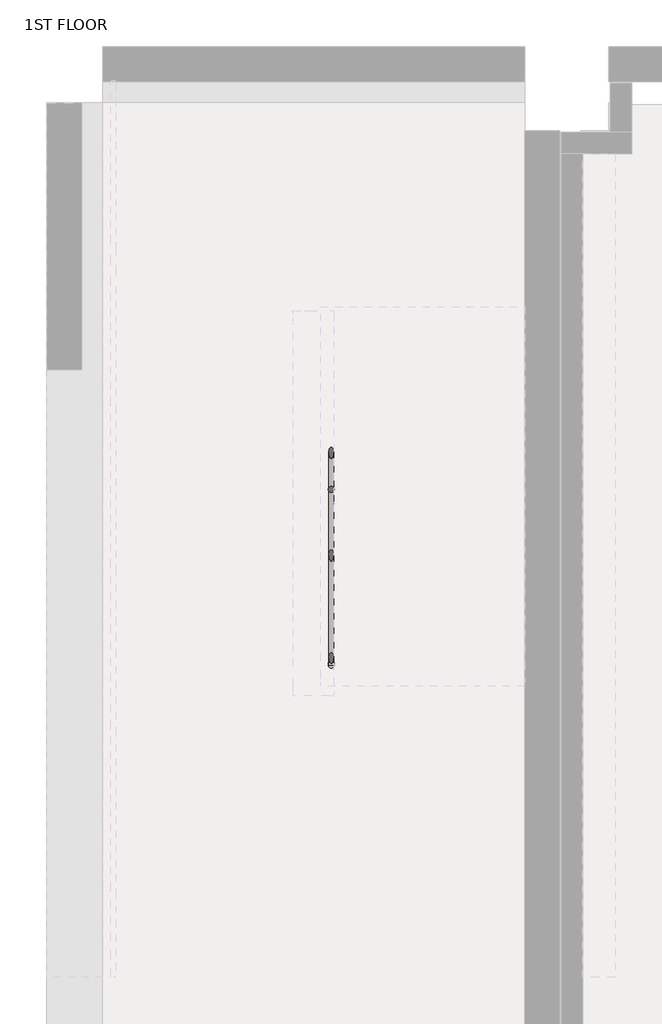
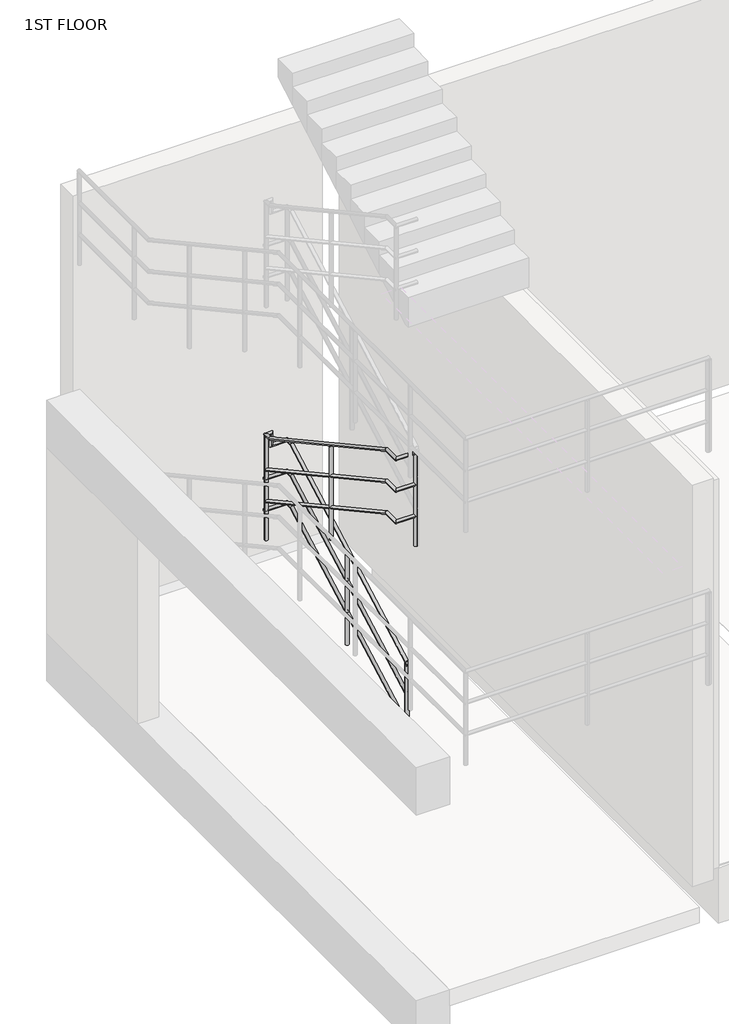
# One storey, part 12 of 15: 1 railing.
"""IFC4 building model written with IfcOpenShell, lengths in millimetres."""

from ifc_helpers import new_model, si_unit, point, frame, frame_2d, origin, place, context, project, spatial, circle_curve, ellipse_curve, trimmed, segment, composite_curve, outline, extrude, element, save
from ifc_brep_helpers import plane_surface, cylinder_surface, advanced_brep

model = new_model("IFC4")

# Units and contexts
model_context = context("Model", 3, world=origin())
ifc_project = project(units=[si_unit("LENGTHUNIT", "METRE", prefix="MILLI")], contexts=[model_context])

# Site, building, storey
site = spatial("IfcSite", under=ifc_project)
building = spatial("IfcBuilding", under=site)
storey = spatial("IfcBuildingStorey", under=building, Name="1ST FLOOR", Elevation=4800.0)

# Railing
placement = place(None, origin())
element("IfcRailing", 1, ObjectType="H_RL_AR_S10_Steel Handrail_H1200_STAIR", at=placement, inside=storey, context=model_context, shape_type="SolidModel", body=[
    advanced_brep(
    [(-1656.0, -4100.0, 5972.7772257), (-1694.0, -4100.0, 5972.7772257), (-1656.0, -1695.134128, 7291.0), (-1694.0, -1695.134128, 7291.0), (-1656.0, -1581.0, 7291.0), (-1694.0, -1619.0, 7291.0), (-1868.0, -1581.0, 7291.0), (-1868.0, -1619.0, 7291.0), (-1868.0, -1581.0, 7442.2888889), (-1868.0, -1619.0, 7442.2888889), (-1944.0, -1581.0, 7442.2888889), (-1906.0, -1619.0, 7442.2888889), (-1944.0, -1680.865872, 7442.2888889), (-1906.0, -1680.865872, 7442.2888889), (-1944.0, -4104.865872, 8771.0), (-1906.0, -4104.865872, 8771.0), (-1944.0, -4319.0, 8771.0), (-1906.0, -4281.0, 8771.0), (-1675.0, -4319.0, 8771.0), (-1675.0, -4281.0, 8771.0)],
    [
        (0, 1, ellipse_curve(frame((-1675.0, -4100.0, 5972.7772257), z_axis=(0.0, -1.0, 0.0), x_axis=(0.0, 0.0, -0.9999999999999999)), 21.6672187, 19.0)),
        (1, 0, ellipse_curve(frame((-1675.0, -4100.0, 5972.7772257), z_axis=(0.0, -1.0, 0.0), x_axis=(0.0, 0.0, -0.9999999999999999)), 21.6672187, 19.0)),
        (0, 2),
        (2, 3, ellipse_curve(frame((-1675.0, -1695.134128, 7291.0), z_axis=(0.0, -0.9687364795192939, -0.24809198545814526), x_axis=(0.0, 0.2480919854581443, -0.9687364795192942)), 19.613177, 19.0)),
        (3, 1),
        (3, 2, ellipse_curve(frame((-1675.0, -1695.134128, 7291.0), z_axis=(0.0, -0.9687364795192939, -0.24809198545814526), x_axis=(0.0, 0.2480919854581443, -0.9687364795192942)), 19.613177, 19.0)),
        (2, 4),
        (4, 5, ellipse_curve(frame((-1675.0, -1600.0, 7291.0), z_axis=(0.7071067811865467, -0.7071067811865485, 0.0), x_axis=(-0.7071067811865485, -0.7071067811865465, 0.0)), 26.8700577, 19.0)),
        (5, 3),
        (5, 4, ellipse_curve(frame((-1675.0, -1600.0, 7291.0), z_axis=(0.7071067811865467, -0.7071067811865485, 0.0), x_axis=(-0.7071067811865485, -0.7071067811865465, 0.0)), 26.8700577, 19.0)),
        (4, 6),
        (6, 7, ellipse_curve(frame((-1868.0, -1600.0, 7291.0), z_axis=(0.7071067811865475, 0.0, -0.7071067811865475), x_axis=(0.7071067811865476, 0.0, 0.7071067811865474)), 26.8700577, 19.0)),
        (7, 5),
        (7, 6, ellipse_curve(frame((-1868.0, -1600.0, 7291.0), z_axis=(0.7071067811865475, 0.0, -0.7071067811865475), x_axis=(0.7071067811865476, 0.0, 0.7071067811865474)), 26.8700577, 19.0)),
        (6, 8),
        (8, 9, ellipse_curve(frame((-1868.0, -1600.0, 7442.2888889), z_axis=(0.7071067811865475, 0.0, -0.7071067811865475), x_axis=(-0.7071067811865474, 0.0, -0.7071067811865476)), 26.8700577, 19.0)),
        (9, 7),
        (9, 8, ellipse_curve(frame((-1868.0, -1600.0, 7442.2888889), z_axis=(0.7071067811865475, 0.0, -0.7071067811865475), x_axis=(-0.7071067811865474, 0.0, -0.7071067811865476)), 26.8700577, 19.0)),
        (8, 10),
        (10, 11, ellipse_curve(frame((-1925.0, -1600.0, 7442.2888889), z_axis=(0.70710678118664, 0.707106781186455, 0.0), x_axis=(0.707106781186455, -0.70710678118664, 0.0)), 26.8700577, 19.0)),
        (11, 9),
        (11, 10, ellipse_curve(frame((-1925.0, -1600.0, 7442.2888889), z_axis=(0.70710678118664, 0.707106781186455, 0.0), x_axis=(0.707106781186455, -0.70710678118664, 0.0)), 26.8700577, 19.0)),
        (10, 12),
        (12, 13, ellipse_curve(frame((-1925.0, -1680.865872, 7442.2888889), z_axis=(0.0, 0.9687364795192939, -0.24809198545814531), x_axis=(0.0, 0.24809198545814604, 0.9687364795192938)), 19.613177, 19.0)),
        (13, 11),
        (13, 12, ellipse_curve(frame((-1925.0, -1680.865872, 7442.2888889), z_axis=(0.0, 0.9687364795192939, -0.24809198545814531), x_axis=(0.0, 0.24809198545814604, 0.9687364795192938)), 19.613177, 19.0)),
        (12, 14),
        (14, 15, ellipse_curve(frame((-1925.0, -4104.865872, 8771.0), z_axis=(0.0, 0.9687364795192939, -0.2480919854581453), x_axis=(0.0, -0.24809198545814418, -0.9687364795192942)), 19.613177, 19.0)),
        (15, 13),
        (15, 14, ellipse_curve(frame((-1925.0, -4104.865872, 8771.0), z_axis=(0.0, 0.9687364795192939, -0.2480919854581453), x_axis=(0.0, -0.24809198545814418, -0.9687364795192942)), 19.613177, 19.0)),
        (14, 16),
        (16, 17, ellipse_curve(frame((-1925.0, -4300.0, 8771.0), z_axis=(-0.7071067811864243, 0.7071067811866708, 0.0), x_axis=(0.7071067811866707, 0.7071067811864242, 0.0)), 26.8700577, 19.0)),
        (17, 15),
        (17, 16, ellipse_curve(frame((-1925.0, -4300.0, 8771.0), z_axis=(-0.7071067811864243, 0.7071067811866708, 0.0), x_axis=(0.7071067811866707, 0.7071067811864242, 0.0)), 26.8700577, 19.0)),
        (18, 19, circle_curve(frame((-1675.0, -4300.0, 8771.0), z_axis=(1.0, 0.0, 0.0), x_axis=(0.0, 1.0, 0.0)), 19.0)),
        (19, 18, circle_curve(frame((-1675.0, -4300.0, 8771.0), z_axis=(1.0, 0.0, 0.0), x_axis=(0.0, 1.0, 0.0)), 19.0)),
        (16, 18),
        (19, 17),
    ],
    [
        plane_surface(frame((-1675.0, -4100.0, 5994.4444444), z_axis=(0.0, -1.0, 0.0), x_axis=(0.0, 0.0, 1.0))),
        cylinder_surface(frame((-1675.0, -4090.8672412, 5977.7833305), z_axis=(0.0, -0.8769007335028709, -0.4806715131793511), x_axis=(-1.0, 0.0, 0.0)), 19.0),
        cylinder_surface(frame((-1675.0, -1700.0, 7291.0), z_axis=(0.0, -1.0, 0.0), x_axis=(-1.0, 0.0, 0.0)), 19.0),
        cylinder_surface(frame((-1675.0, -1600.0, 7291.0), z_axis=(1.0, 0.0, 0.0), x_axis=(0.0, -1.0, 0.0)), 19.0),
        cylinder_surface(frame((-1868.0, -1600.0, 7310.0), z_axis=(0.0, 0.0, -1.0), x_axis=(0.0, -1.0, 0.0)), 19.0),
        cylinder_surface(frame((-1849.0, -1600.0, 7442.2888889), z_axis=(1.0, 0.0, 0.0), x_axis=(0.0, -1.0, 0.0)), 19.0),
        cylinder_surface(frame((-1925.0, -1600.0, 7442.2888889), z_axis=(0.0, 1.0, 0.0), x_axis=(1.0, 0.0, 0.0)), 19.0),
        cylinder_surface(frame((-1925.0, -1685.1327588, 7444.627775), z_axis=(0.0, 0.8769007335028708, -0.4806715131793512), x_axis=(1.0, 0.0, 0.0)), 19.0),
        cylinder_surface(frame((-1925.0, -4100.0, 8771.0), z_axis=(0.0, 1.0, 0.0), x_axis=(1.0, 0.0, 0.0)), 19.0),
        plane_surface(frame((-1675.0, -4300.0, 8790.0), z_axis=(1.0, 0.0, 0.0), x_axis=(0.0, 1.0, 0.0))),
        cylinder_surface(frame((-1925.0, -4300.0, 8771.0), z_axis=(-1.0, 0.0, 0.0), x_axis=(0.0, 1.0, 0.0)), 19.0),
    ],
    [
        (0, [[1, 2]]),
        (1, [[-1, 3, 4, 5]]),
        (1, [[-2, -5, 6, -3]]),
        (2, [[-4, 7, 8, 9]]),
        (2, [[-6, -9, 10, -7]]),
        (3, [[-8, 11, 12, 13]]),
        (3, [[-10, -13, 14, -11]]),
        (4, [[-12, 15, 16, 17]]),
        (4, [[-14, -17, 18, -15]]),
        (5, [[-16, 19, 20, 21]]),
        (5, [[-18, -21, 22, -19]]),
        (6, [[-20, 23, 24, 25]]),
        (6, [[-22, -25, 26, -23]]),
        (7, [[-24, 27, 28, 29]]),
        (7, [[-26, -29, 30, -27]]),
        (8, [[-28, 31, 32, 33]]),
        (8, [[-30, -33, 34, -31]]),
        (9, [[35, 36]]),
        (10, [[-32, 37, -36, 38]]),
        (10, [[-34, -38, -35, -37]]),
    ],
),
    advanced_brep(
    [(-1675.0, -4319.0, 7971.0), (-1675.0, -4281.0, 7971.0), (-1944.0, -4319.0, 7971.0), (-1906.0, -4281.0, 7971.0)],
    [
        (0, 1, circle_curve(frame((-1675.0, -4300.0, 7971.0), z_axis=(1.0, 0.0, 0.0), x_axis=(0.0, 1.0, 0.0)), 19.0)),
        (1, 0, circle_curve(frame((-1675.0, -4300.0, 7971.0), z_axis=(1.0, 0.0, 0.0), x_axis=(0.0, 1.0, 0.0)), 19.0)),
        (2, 3, ellipse_curve(frame((-1925.0, -4300.0, 7971.0), z_axis=(-0.7071067811865471, 0.7071067811865479, 0.0), x_axis=(0.7071067811865479, 0.7071067811865471, 0.0)), 26.8700577, 19.0)),
        (3, 2, ellipse_curve(frame((-1925.0, -4300.0, 7971.0), z_axis=(-0.7071067811865471, 0.7071067811865479, 0.0), x_axis=(0.7071067811865479, 0.7071067811865471, 0.0)), 26.8700577, 19.0)),
        (0, 2),
        (3, 1),
    ],
    [
        plane_surface(frame((-1675.0, -4300.0, 7990.0), z_axis=(1.0, 0.0, 0.0), x_axis=(0.0, -1.0, 0.0))),
        plane_surface(frame((-1925.0, -4300.0, 7990.0), z_axis=(-0.7071067811865471, 0.7071067811865479, 0.0), x_axis=(0.7071067811865479, 0.7071067811865471, 0.0))),
        cylinder_surface(frame((-1675.0, -4300.0, 7971.0), z_axis=(1.0, 0.0, 0.0), x_axis=(0.0, 1.0, 0.0)), 19.0),
    ],
    [
        (0, [[1, 2]]),
        (1, [[3, 4]]),
        (2, [[-1, 5, -4, 6]]),
        (2, [[-2, -6, -3, -5]]),
    ],
),
    advanced_brep(
    [(-1944.0, -4319.0, 7971.0), (-1906.0, -4281.0, 7971.0), (-1944.0, -4104.865872, 7971.0), (-1906.0, -4104.865872, 7971.0), (-1944.0, -1592.4716448, 6593.8357569), (-1906.0, -1625.7938727, 6612.1012744)],
    [
        (0, 1, ellipse_curve(frame((-1925.0, -4300.0, 7971.0), z_axis=(0.7071067811865471, -0.7071067811865479, 0.0), x_axis=(-0.7071067811865478, -0.7071067811865472, 0.0)), 26.8700577, 19.0)),
        (1, 0, ellipse_curve(frame((-1925.0, -4300.0, 7971.0), z_axis=(0.7071067811865471, -0.7071067811865479, 0.0), x_axis=(-0.7071067811865478, -0.7071067811865472, 0.0)), 26.8700577, 19.0)),
        (0, 2),
        (2, 3, ellipse_curve(frame((-1925.0, -4104.865872, 7971.0), z_axis=(0.0, -0.9687364795192939, 0.24809198545814531), x_axis=(0.0, -0.24809198545814604, -0.9687364795192938)), 19.613177, 19.0)),
        (3, 1),
        (3, 2, ellipse_curve(frame((-1925.0, -4104.865872, 7971.0), z_axis=(0.0, -0.9687364795192939, 0.24809198545814531), x_axis=(0.0, -0.24809198545814604, -0.9687364795192938)), 19.613177, 19.0)),
        (4, 5, ellipse_curve(frame((-1925.0, -1609.1327588, 6602.9685157), z_axis=(0.7071067811865346, 0.6200624550873559, -0.33988608649231156), x_axis=(0.7071067811865606, -0.6200624550873189, 0.33988608649232477)), 26.8700577, 19.0)),
        (5, 4, ellipse_curve(frame((-1925.0, -1609.1327588, 6602.9685157), z_axis=(0.7071067811865346, 0.6200624550873559, -0.33988608649231156), x_axis=(0.7071067811865606, -0.6200624550873189, 0.33988608649232477)), 26.8700577, 19.0)),
        (2, 4),
        (5, 3),
    ],
    [
        plane_surface(frame((-1925.0, -4300.0, 7990.0), z_axis=(0.7071067811865471, -0.7071067811865479, 0.0), x_axis=(0.7071067811865479, 0.7071067811865471, 0.0))),
        cylinder_surface(frame((-1925.0, -4300.0, 7971.0), z_axis=(0.0, -1.0, 0.0), x_axis=(1.0, 0.0, 0.0)), 19.0),
        plane_surface(frame((-1925.0, -1600.0, 6619.6296296), z_axis=(0.7071067811865346, 0.6200624550873559, -0.33988608649231156), x_axis=(0.7071067811865605, -0.6200624550873332, 0.33988608649229907))),
        cylinder_surface(frame((-1925.0, -4109.1327588, 7973.3388861), z_axis=(0.0, -0.8769007335028708, 0.4806715131793512), x_axis=(1.0, 0.0, 0.0)), 19.0),
    ],
    [
        (0, [[1, 2]]),
        (1, [[-1, 3, 4, 5]]),
        (1, [[-2, -5, 6, -3]]),
        (2, [[7, 8]]),
        (3, [[-4, 9, -8, 10]]),
        (3, [[-6, -10, -7, -9]]),
    ],
),
    advanced_brep(
    [(-1950.7938727, -1581.0, 6491.0), (-1917.4716448, -1619.0, 6491.0), (-1656.0, -1581.0, 6491.0), (-1694.0, -1619.0, 6491.0)],
    [
        (0, 1, ellipse_curve(frame((-1934.1327587, -1600.0, 6491.0), z_axis=(-0.7071067811865346, -0.6200624550873559, 0.33988608649231156), x_axis=(-0.7071067811865603, 0.6200624550873332, -0.33988608649229907)), 26.8700577, 19.0)),
        (1, 0, ellipse_curve(frame((-1934.1327587, -1600.0, 6491.0), z_axis=(-0.7071067811865346, -0.6200624550873559, 0.33988608649231156), x_axis=(-0.7071067811865603, 0.6200624550873332, -0.33988608649229907)), 26.8700577, 19.0)),
        (2, 3, ellipse_curve(frame((-1675.0, -1600.0, 6491.0), z_axis=(0.7071067811865619, -0.7071067811865331, 0.0), x_axis=(-0.7071067811865331, -0.7071067811865619, 0.0)), 26.8700577, 19.0)),
        (3, 2, ellipse_curve(frame((-1675.0, -1600.0, 6491.0), z_axis=(0.7071067811865619, -0.7071067811865331, 0.0), x_axis=(-0.7071067811865331, -0.7071067811865619, 0.0)), 26.8700577, 19.0)),
        (0, 2),
        (3, 1),
    ],
    [
        plane_surface(frame((-1925.0, -1600.0, 6510.0), z_axis=(-0.7071067811865346, -0.6200624550873559, 0.33988608649231156), x_axis=(0.7071067811865605, -0.6200624550873332, 0.33988608649229907))),
        plane_surface(frame((-1675.0, -1600.0, 6510.0), z_axis=(0.7071067811865619, -0.7071067811865331, 0.0), x_axis=(0.7071067811865331, 0.7071067811865619, 0.0))),
        cylinder_surface(frame((-1925.0, -1600.0, 6491.0), z_axis=(-1.0, 0.0, 0.0), x_axis=(0.0, -1.0, 0.0)), 19.0),
    ],
    [
        (0, [[1, 2]]),
        (1, [[3, 4]]),
        (2, [[-1, 5, -4, 6]]),
        (2, [[-2, -6, -3, -5]]),
    ],
),
    advanced_brep(
    [(-1656.0, -1581.0, 6491.0), (-1694.0, -1619.0, 6491.0), (-1656.0, -1695.134128, 6491.0), (-1694.0, -1695.134128, 6491.0), (-1656.0, -4100.0, 5172.7772257), (-1694.0, -4100.0, 5172.7772257)],
    [
        (0, 1, ellipse_curve(frame((-1675.0, -1600.0, 6491.0), z_axis=(-0.7071067811865619, 0.7071067811865331, 0.0), x_axis=(0.707106781186533, 0.7071067811865619, 0.0)), 26.8700577, 19.0)),
        (1, 0, ellipse_curve(frame((-1675.0, -1600.0, 6491.0), z_axis=(-0.7071067811865619, 0.7071067811865331, 0.0), x_axis=(0.707106781186533, 0.7071067811865619, 0.0)), 26.8700577, 19.0)),
        (0, 2),
        (2, 3, ellipse_curve(frame((-1675.0, -1695.134128, 6491.0), z_axis=(0.0, 0.9687364795192939, 0.24809198545814526), x_axis=(0.0, 0.2480919854581461, -0.9687364795192938)), 19.613177, 19.0)),
        (3, 1),
        (3, 2, ellipse_curve(frame((-1675.0, -1695.134128, 6491.0), z_axis=(0.0, 0.9687364795192939, 0.24809198545814526), x_axis=(0.0, 0.2480919854581461, -0.9687364795192938)), 19.613177, 19.0)),
        (4, 5, ellipse_curve(frame((-1675.0, -4100.0, 5172.7772257), z_axis=(0.0, -1.0, 0.0), x_axis=(0.0, 0.0, 0.9999999999999999)), 21.6672187, 19.0)),
        (5, 4, ellipse_curve(frame((-1675.0, -4100.0, 5172.7772257), z_axis=(0.0, -1.0, 0.0), x_axis=(0.0, 0.0, 0.9999999999999999)), 21.6672187, 19.0)),
        (2, 4),
        (5, 3),
    ],
    [
        plane_surface(frame((-1675.0, -1600.0, 6510.0), z_axis=(-0.7071067811865619, 0.7071067811865331, 0.0), x_axis=(0.7071067811865331, 0.7071067811865619, 0.0))),
        cylinder_surface(frame((-1675.0, -1600.0, 6491.0), z_axis=(0.0, 1.0, 0.0), x_axis=(-1.0, 0.0, 0.0)), 19.0),
        plane_surface(frame((-1675.0, -4100.0, 5194.4444444), z_axis=(0.0, -1.0, 0.0), x_axis=(0.0, 0.0, -1.0))),
        cylinder_surface(frame((-1675.0, -1690.8672412, 6493.3388861), z_axis=(0.0, 0.8769007335028709, 0.4806715131793511), x_axis=(-1.0, 0.0, 0.0)), 19.0),
    ],
    [
        (0, [[1, 2]]),
        (1, [[-1, 3, 4, 5]]),
        (1, [[-2, -5, 6, -3]]),
        (2, [[7, 8]]),
        (3, [[-4, 9, -8, 10]]),
        (3, [[-6, -10, -7, -9]]),
    ],
),
    advanced_brep(
    [(-1675.0, -4319.0, 8371.0), (-1675.0, -4281.0, 8371.0), (-1944.0, -4319.0, 8371.0), (-1906.0, -4281.0, 8371.0)],
    [
        (0, 1, circle_curve(frame((-1675.0, -4300.0, 8371.0), z_axis=(1.0, 0.0, 0.0), x_axis=(0.0, 1.0, 0.0)), 19.0)),
        (1, 0, circle_curve(frame((-1675.0, -4300.0, 8371.0), z_axis=(1.0, 0.0, 0.0), x_axis=(0.0, 1.0, 0.0)), 19.0)),
        (2, 3, ellipse_curve(frame((-1925.0, -4300.0, 8371.0), z_axis=(-0.7071067811865471, 0.7071067811865479, 0.0), x_axis=(0.7071067811865479, 0.7071067811865471, 0.0)), 26.8700577, 19.0)),
        (3, 2, ellipse_curve(frame((-1925.0, -4300.0, 8371.0), z_axis=(-0.7071067811865471, 0.7071067811865479, 0.0), x_axis=(0.7071067811865479, 0.7071067811865471, 0.0)), 26.8700577, 19.0)),
        (0, 2),
        (3, 1),
    ],
    [
        plane_surface(frame((-1675.0, -4300.0, 8390.0), z_axis=(1.0, 0.0, 0.0), x_axis=(0.0, -1.0, 0.0))),
        plane_surface(frame((-1925.0, -4300.0, 8390.0), z_axis=(-0.7071067811865471, 0.7071067811865479, 0.0), x_axis=(0.7071067811865479, 0.7071067811865471, 0.0))),
        cylinder_surface(frame((-1675.0, -4300.0, 8371.0), z_axis=(1.0, 0.0, 0.0), x_axis=(0.0, 1.0, 0.0)), 19.0),
    ],
    [
        (0, [[1, 2]]),
        (1, [[3, 4]]),
        (2, [[-1, 5, -4, 6]]),
        (2, [[-2, -6, -3, -5]]),
    ],
),
    advanced_brep(
    [(-1944.0, -4319.0, 8371.0), (-1906.0, -4281.0, 8371.0), (-1944.0, -4104.865872, 8371.0), (-1906.0, -4104.865872, 8371.0), (-1944.0, -1592.4716448, 6993.8357569), (-1906.0, -1625.7938727, 7012.1012744)],
    [
        (0, 1, ellipse_curve(frame((-1925.0, -4300.0, 8371.0), z_axis=(0.7071067811865471, -0.7071067811865479, 0.0), x_axis=(-0.7071067811865478, -0.7071067811865472, 0.0)), 26.8700577, 19.0)),
        (1, 0, ellipse_curve(frame((-1925.0, -4300.0, 8371.0), z_axis=(0.7071067811865471, -0.7071067811865479, 0.0), x_axis=(-0.7071067811865478, -0.7071067811865472, 0.0)), 26.8700577, 19.0)),
        (0, 2),
        (2, 3, ellipse_curve(frame((-1925.0, -4104.865872, 8371.0), z_axis=(0.0, -0.9687364795192939, 0.24809198545814531), x_axis=(0.0, -0.24809198545814604, -0.9687364795192938)), 19.613177, 19.0)),
        (3, 1),
        (3, 2, ellipse_curve(frame((-1925.0, -4104.865872, 8371.0), z_axis=(0.0, -0.9687364795192939, 0.24809198545814531), x_axis=(0.0, -0.24809198545814604, -0.9687364795192938)), 19.613177, 19.0)),
        (4, 5, ellipse_curve(frame((-1925.0, -1609.1327588, 7002.9685157), z_axis=(0.7071067811865346, 0.6200624550873559, -0.33988608649231156), x_axis=(0.7071067811865606, -0.6200624550873189, 0.33988608649232477)), 26.8700577, 19.0)),
        (5, 4, ellipse_curve(frame((-1925.0, -1609.1327588, 7002.9685157), z_axis=(0.7071067811865346, 0.6200624550873559, -0.33988608649231156), x_axis=(0.7071067811865606, -0.6200624550873189, 0.33988608649232477)), 26.8700577, 19.0)),
        (2, 4),
        (5, 3),
    ],
    [
        plane_surface(frame((-1925.0, -4300.0, 8390.0), z_axis=(0.7071067811865471, -0.7071067811865479, 0.0), x_axis=(0.7071067811865479, 0.7071067811865471, 0.0))),
        cylinder_surface(frame((-1925.0, -4300.0, 8371.0), z_axis=(0.0, -1.0, 0.0), x_axis=(1.0, 0.0, 0.0)), 19.0),
        plane_surface(frame((-1925.0, -1600.0, 7019.6296296), z_axis=(0.7071067811865346, 0.6200624550873559, -0.33988608649231156), x_axis=(0.7071067811865605, -0.6200624550873332, 0.33988608649229907))),
        cylinder_surface(frame((-1925.0, -4109.1327588, 8373.3388861), z_axis=(0.0, -0.8769007335028708, 0.4806715131793512), x_axis=(1.0, 0.0, 0.0)), 19.0),
    ],
    [
        (0, [[1, 2]]),
        (1, [[-1, 3, 4, 5]]),
        (1, [[-2, -5, 6, -3]]),
        (2, [[7, 8]]),
        (3, [[-4, 9, -8, 10]]),
        (3, [[-6, -10, -7, -9]]),
    ],
),
    advanced_brep(
    [(-1950.7938727, -1581.0, 6891.0), (-1917.4716448, -1619.0, 6891.0), (-1656.0, -1581.0, 6891.0), (-1694.0, -1619.0, 6891.0)],
    [
        (0, 1, ellipse_curve(frame((-1934.1327587, -1600.0, 6891.0), z_axis=(-0.7071067811865346, -0.6200624550873559, 0.33988608649231156), x_axis=(-0.7071067811865603, 0.6200624550873332, -0.33988608649229907)), 26.8700577, 19.0)),
        (1, 0, ellipse_curve(frame((-1934.1327587, -1600.0, 6891.0), z_axis=(-0.7071067811865346, -0.6200624550873559, 0.33988608649231156), x_axis=(-0.7071067811865603, 0.6200624550873332, -0.33988608649229907)), 26.8700577, 19.0)),
        (2, 3, ellipse_curve(frame((-1675.0, -1600.0, 6891.0), z_axis=(0.7071067811865619, -0.7071067811865331, 0.0), x_axis=(-0.7071067811865331, -0.7071067811865619, 0.0)), 26.8700577, 19.0)),
        (3, 2, ellipse_curve(frame((-1675.0, -1600.0, 6891.0), z_axis=(0.7071067811865619, -0.7071067811865331, 0.0), x_axis=(-0.7071067811865331, -0.7071067811865619, 0.0)), 26.8700577, 19.0)),
        (0, 2),
        (3, 1),
    ],
    [
        plane_surface(frame((-1925.0, -1600.0, 6910.0), z_axis=(-0.7071067811865346, -0.6200624550873559, 0.33988608649231156), x_axis=(0.7071067811865605, -0.6200624550873332, 0.33988608649229907))),
        plane_surface(frame((-1675.0, -1600.0, 6910.0), z_axis=(0.7071067811865619, -0.7071067811865331, 0.0), x_axis=(0.7071067811865331, 0.7071067811865619, 0.0))),
        cylinder_surface(frame((-1925.0, -1600.0, 6891.0), z_axis=(-1.0, 0.0, 0.0), x_axis=(0.0, -1.0, 0.0)), 19.0),
    ],
    [
        (0, [[1, 2]]),
        (1, [[3, 4]]),
        (2, [[-1, 5, -4, 6]]),
        (2, [[-2, -6, -3, -5]]),
    ],
),
    advanced_brep(
    [(-1656.0, -1581.0, 6891.0), (-1694.0, -1619.0, 6891.0), (-1656.0, -1695.134128, 6891.0), (-1694.0, -1695.134128, 6891.0), (-1656.0, -4100.0, 5572.7772257), (-1694.0, -4100.0, 5572.7772257)],
    [
        (0, 1, ellipse_curve(frame((-1675.0, -1600.0, 6891.0), z_axis=(-0.7071067811865619, 0.7071067811865331, 0.0), x_axis=(0.707106781186533, 0.7071067811865619, 0.0)), 26.8700577, 19.0)),
        (1, 0, ellipse_curve(frame((-1675.0, -1600.0, 6891.0), z_axis=(-0.7071067811865619, 0.7071067811865331, 0.0), x_axis=(0.707106781186533, 0.7071067811865619, 0.0)), 26.8700577, 19.0)),
        (0, 2),
        (2, 3, ellipse_curve(frame((-1675.0, -1695.134128, 6891.0), z_axis=(0.0, 0.9687364795192939, 0.24809198545814526), x_axis=(0.0, 0.2480919854581461, -0.9687364795192938)), 19.613177, 19.0)),
        (3, 1),
        (3, 2, ellipse_curve(frame((-1675.0, -1695.134128, 6891.0), z_axis=(0.0, 0.9687364795192939, 0.24809198545814526), x_axis=(0.0, 0.2480919854581461, -0.9687364795192938)), 19.613177, 19.0)),
        (4, 5, ellipse_curve(frame((-1675.0, -4100.0, 5572.7772257), z_axis=(0.0, -1.0, 0.0), x_axis=(0.0, 0.0, 0.9999999999999999)), 21.6672187, 19.0)),
        (5, 4, ellipse_curve(frame((-1675.0, -4100.0, 5572.7772257), z_axis=(0.0, -1.0, 0.0), x_axis=(0.0, 0.0, 0.9999999999999999)), 21.6672187, 19.0)),
        (2, 4),
        (5, 3),
    ],
    [
        plane_surface(frame((-1675.0, -1600.0, 6910.0), z_axis=(-0.7071067811865619, 0.7071067811865331, 0.0), x_axis=(0.7071067811865331, 0.7071067811865619, 0.0))),
        cylinder_surface(frame((-1675.0, -1600.0, 6891.0), z_axis=(0.0, 1.0, 0.0), x_axis=(-1.0, 0.0, 0.0)), 19.0),
        plane_surface(frame((-1675.0, -4100.0, 5594.4444444), z_axis=(0.0, -1.0, 0.0), x_axis=(0.0, 0.0, -1.0))),
        cylinder_surface(frame((-1675.0, -1690.8672412, 6893.3388861), z_axis=(0.0, 0.8769007335028709, 0.4806715131793511), x_axis=(-1.0, 0.0, 0.0)), 19.0),
    ],
    [
        (0, [[1, 2]]),
        (1, [[-1, 3, 4, 5]]),
        (1, [[-2, -5, 6, -3]]),
        (2, [[7, 8]]),
        (3, [[-4, 9, -8, 10]]),
        (3, [[-6, -10, -7, -9]]),
    ],
),
    advanced_brep(
    [(-1696.2, -4100.0, 5951.110007), (-1696.2, -4100.0, 4794.4444444), (-1653.8, -4100.0, 4794.4444444), (-1653.8, -4100.0, 5951.110007)],
    [
        (0, 1),
        (1, 2, circle_curve(frame((-1675.0, -4100.0, 4794.4444444), z_axis=(0.0, 0.0, 1.0), x_axis=(1.0, 0.0, 0.0)), 21.2)),
        (2, 3),
        (3, 0, ellipse_curve(frame((-1675.0, -4100.0, 5951.110007), z_axis=(0.0, 0.4806715131793496, -0.8769007335028717), x_axis=(0.0, 0.8769007335028718, 0.4806715131793496)), 24.1760546, 21.2)),
        (0, 3, ellipse_curve(frame((-1675.0, -4100.0, 5951.110007), z_axis=(0.0, 0.4806715131793496, -0.8769007335028717), x_axis=(0.0, 0.8769007335028718, 0.4806715131793496)), 24.1760546, 21.2)),
        (2, 1, circle_curve(frame((-1675.0, -4100.0, 4794.4444444), z_axis=(0.0, 0.0, 1.0), x_axis=(1.0, 0.0, 0.0)), 21.2)),
    ],
    [
        cylinder_surface(frame((-1675.0, -4100.0, 4694.4444444), z_axis=(0.0, 0.0, 1.0), x_axis=(1.0, 0.0, 0.0)), 21.2),
        plane_surface(frame((-1650.0, -4125.0, 5937.4063033), z_axis=(0.0, -0.4806715131793496, 0.8769007335028717), x_axis=(-1.0, 0.0, 0.0))),
        plane_surface(frame((-1650.0, -4075.0, 4794.4444444), z_axis=(0.0, 0.0, -1.0), x_axis=(-1.0, 0.0, 0.0))),
    ],
    [
        (0, [[1, 2, 3, 4]]),
        (0, [[-1, 5, -3, 6]]),
        (1, [[-4, -5]]),
        (2, [[-2, -6]]),
    ],
),
    advanced_brep(
    [(-1696.2, -2850.0, 6636.2951922), (-1696.2, -2850.0, 5452.2222222), (-1653.8, -2850.0, 5452.2222222), (-1653.8, -2850.0, 6636.2951922)],
    [
        (0, 1),
        (1, 2, circle_curve(frame((-1675.0, -2850.0, 5452.2222222), z_axis=(0.0, 0.0, 1.0), x_axis=(1.0, 0.0, 0.0)), 21.2)),
        (2, 3),
        (3, 0, ellipse_curve(frame((-1675.0, -2850.0, 6636.2951922), z_axis=(0.0, 0.4806715131793478, -0.8769007335028728), x_axis=(0.0, 0.8769007335028729, 0.4806715131793474)), 24.1760546, 21.2)),
        (0, 3, ellipse_curve(frame((-1675.0, -2850.0, 6636.2951922), z_axis=(0.0, 0.4806715131793478, -0.8769007335028728), x_axis=(0.0, 0.8769007335028729, 0.4806715131793474)), 24.1760546, 21.2)),
        (2, 1, circle_curve(frame((-1675.0, -2850.0, 5452.2222222), z_axis=(0.0, 0.0, 1.0), x_axis=(1.0, 0.0, 0.0)), 21.2)),
    ],
    [
        cylinder_surface(frame((-1675.0, -2850.0, 5352.2222222), z_axis=(0.0, 0.0, 1.0), x_axis=(1.0, 0.0, 0.0)), 21.2),
        plane_surface(frame((-1650.0, -2875.0, 6622.5914885), z_axis=(0.0, -0.4806715131793478, 0.8769007335028728), x_axis=(-1.0, 0.0, 0.0))),
        plane_surface(frame((-1650.0, -2825.0, 5452.2222222), z_axis=(0.0, 0.0, -1.0), x_axis=(-1.0, 0.0, 0.0))),
    ],
    [
        (0, [[1, 2, 3, 4]]),
        (0, [[-1, 5, -3, 6]]),
        (1, [[-4, -5]]),
        (2, [[-2, -6]]),
    ],
),
    extrude(outline(composite_curve([segment(trimmed(circle_curve(frame_2d((-1925.0, -1600.0)), 21.2), [point((-1946.2, -1600.0))], [point((-1903.8, -1600.0))], False, "CARTESIAN"), True, "CONTINUOUS"), segment(trimmed(circle_curve(frame_2d((-1925.0, -1600.0)), 21.2), [point((-1903.8, -1600.0))], [point((-1946.2, -1600.0))], False, "CARTESIAN"), True, "CONTINUOUS")], self_intersect=False)), frame((0.0, 0.0, 6110.0), z_axis=(0.0, 0.0, 1.0), x_axis=(1.0, 0.0, 0.0)), (0.0, 0.0, 1.0), 1313.2888889),
    advanced_brep(
    [(-1903.8, -2950.0, 8116.2951922), (-1903.8, -2950.0, 6932.2222222), (-1946.2, -2950.0, 6932.2222222), (-1946.2, -2950.0, 8116.2951922)],
    [
        (0, 1),
        (1, 2, circle_curve(frame((-1925.0, -2950.0, 6932.2222222), z_axis=(0.0, 0.0, 1.0), x_axis=(-1.0, 0.0, 0.0)), 21.2)),
        (2, 3),
        (3, 0, ellipse_curve(frame((-1925.0, -2950.0, 8116.2951922), z_axis=(0.0, -0.4806715131793478, -0.8769007335028728), x_axis=(0.0, -0.8769007335028729, 0.4806715131793474)), 24.1760546, 21.2)),
        (0, 3, ellipse_curve(frame((-1925.0, -2950.0, 8116.2951922), z_axis=(0.0, -0.4806715131793478, -0.8769007335028728), x_axis=(0.0, -0.8769007335028729, 0.4806715131793474)), 24.1760546, 21.2)),
        (2, 1, circle_curve(frame((-1925.0, -2950.0, 6932.2222222), z_axis=(0.0, 0.0, 1.0), x_axis=(-1.0, 0.0, 0.0)), 21.2)),
    ],
    [
        cylinder_surface(frame((-1925.0, -2950.0, 6832.2222222), z_axis=(0.0, 0.0, 1.0), x_axis=(-1.0, 0.0, 0.0)), 21.2),
        plane_surface(frame((-1950.0, -2925.0, 8102.5914885), z_axis=(0.0, 0.4806715131793478, 0.8769007335028728), x_axis=(1.0, 0.0, 0.0))),
        plane_surface(frame((-1950.0, -2975.0, 6932.2222222), z_axis=(0.0, 0.0, -1.0), x_axis=(1.0, 0.0, 0.0))),
    ],
    [
        (0, [[1, 2, 3, 4]]),
        (0, [[-1, 5, -3, 6]]),
        (1, [[-4, -5]]),
        (2, [[-2, -6]]),
    ],
),
    advanced_brep(
    [(-1696.2, -4087.5, 5957.9618588), (-1696.2, -4087.5, 4794.4444444), (-1653.8, -4087.5, 4794.4444444), (-1653.8, -4087.5, 5957.9618588)],
    [
        (0, 1),
        (1, 2, circle_curve(frame((-1675.0, -4087.5, 4794.4444444), z_axis=(0.0, 0.0, 1.0), x_axis=(1.0, 0.0, 0.0)), 21.2)),
        (2, 3),
        (3, 0, ellipse_curve(frame((-1675.0, -4087.5, 5957.9618588), z_axis=(0.0, 0.4806715131793478, -0.8769007335028728), x_axis=(0.0, 0.8769007335028729, 0.4806715131793474)), 24.1760546, 21.2)),
        (0, 3, ellipse_curve(frame((-1675.0, -4087.5, 5957.9618588), z_axis=(0.0, 0.4806715131793478, -0.8769007335028728), x_axis=(0.0, 0.8769007335028729, 0.4806715131793474)), 24.1760546, 21.2)),
        (2, 1, circle_curve(frame((-1675.0, -4087.5, 4794.4444444), z_axis=(0.0, 0.0, 1.0), x_axis=(1.0, 0.0, 0.0)), 21.2)),
    ],
    [
        cylinder_surface(frame((-1675.0, -4087.5, 4694.4444444), z_axis=(0.0, 0.0, 1.0), x_axis=(1.0, 0.0, 0.0)), 21.2),
        plane_surface(frame((-1650.0, -4112.5, 5944.2581551), z_axis=(0.0, -0.4806715131793478, 0.8769007335028728), x_axis=(-1.0, 0.0, 0.0))),
        plane_surface(frame((-1650.0, -4062.5, 4794.4444444), z_axis=(0.0, 0.0, -1.0), x_axis=(-1.0, 0.0, 0.0))),
    ],
    [
        (0, [[1, 2, 3, 4]]),
        (0, [[-1, 5, -3, 6]]),
        (1, [[-4, -5]]),
        (2, [[-2, -6]]),
    ],
),
    extrude(outline(composite_curve([segment(trimmed(circle_curve(frame_2d((-1687.5, -4300.0)), 21.2), [point((-1687.5, -4321.2))], [point((-1687.5, -4278.8))], False, "CARTESIAN"), True, "CONTINUOUS"), segment(trimmed(circle_curve(frame_2d((-1687.5, -4300.0)), 21.2), [point((-1687.5, -4278.8))], [point((-1687.5, -4321.2))], False, "CARTESIAN"), True, "CONTINUOUS")], self_intersect=False)), frame((0.0, 0.0, 7590.0), z_axis=(0.0, 0.0, 1.0), x_axis=(1.0, 0.0, 0.0)), (0.0, 0.0, 1.0), 1162.0),
])

save(model, "model.ifc")

# Revit data of these elements
# Type "H_RL_AR_S10_Steel Handrail_H1200_STAIR"
#   built-in parameter 1008612 = 0.166667 (stored number, unit not read)
#   built-in parameter 1008611 = 0.166667 (stored number, unit not read)
#   built-in parameter 1008609 = 0.459318 (stored number, unit not read)
#   built-in parameter 1008604 = 0.25 (stored number, unit not read)
#   built-in parameter 1008603 = 0.166667 (stored number, unit not read)
#   Railing Height = 1200 mm
#   built-in parameter 1008632 = 1
#   built-in parameter 1008610 = 1
#   built-in parameter 1008618 = M_Baluster - Square : 25mm
# Element 1 (IfcRailing, "H_RL_AR_S10_Steel Handrail_H1200_STAIR")
#   built-in parameter 1008621 = 0.360892 (stored number, unit not read)
#   Phase Created = New Construction
